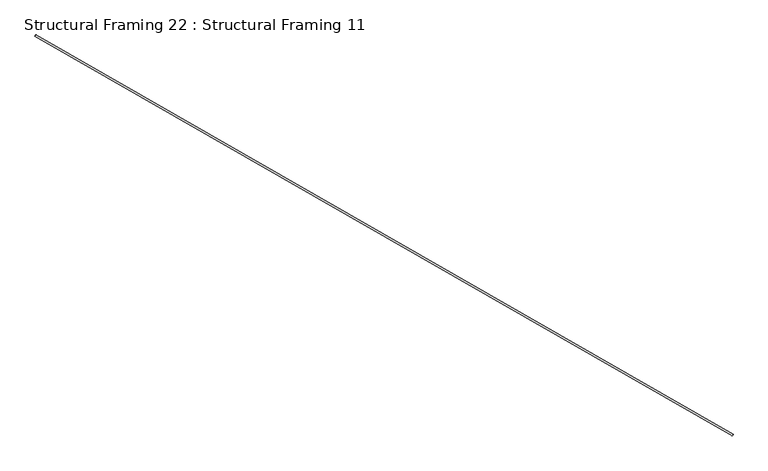
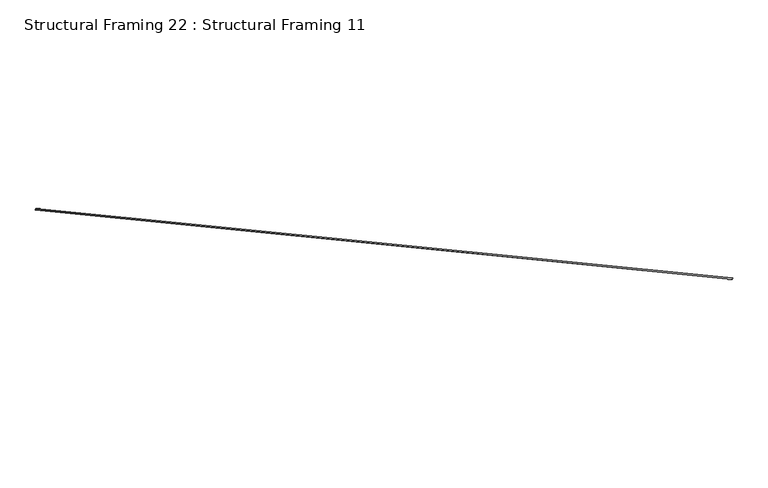
"""IFC4 building model written with IfcOpenShell, lengths in millimetres: beam geometry, Structural Framing 22 : Structural Framing 11."""

from ifc_helpers import new_model, si_unit, point, frame, origin, origin_2d, place, context, project, spatial, circle_curve, trimmed, segment, composite_curve, outline, extrude, source, transform, mapped, element, save


def structural_framing_22_structural_framing_11_913bd44a(model_context):
    return source(origin(), model_context, "Body", "SweptSolid", [
        extrude(outline(composite_curve([segment(trimmed(circle_curve(origin_2d(), 6.35), [point((0.0, -6.35))], [point((0.0, 6.35))], False, "CARTESIAN"), True, "CONTINUOUS"), segment(trimmed(circle_curve(origin_2d(), 6.35), [point((0.0, 6.35))], [point((0.0, -6.35))], False, "CARTESIAN"), True, "CONTINUOUS")], self_intersect=False)), frame((28346.1075052, 4180.6567775, 4935.1357581), z_axis=(-0.8608596592499228, 0.49364969439625245, 0.12341242359905888), x_axis=(0.0, -0.24253562503632656, 0.9701425001453335)), (0.0, 0.0, 1.0), 5892.4476777),
    ])


if __name__ == "__main__":
    model = new_model("IFC4")
    model_context = context("Model", 3, world=origin())
    ifc_project = project(units=[si_unit("LENGTHUNIT", "METRE", prefix="MILLI")], contexts=[model_context])
    site = spatial("IfcSite", under=ifc_project)
    building = spatial("IfcBuilding", under=site)
    placement = place(None, origin())
    structural_framing_22_structural_framing_11_shape = structural_framing_22_structural_framing_11_913bd44a(model_context)
    element("IfcBeam", 1, ObjectType="Structural Framing 22 : Structural Framing 11", at=placement, inside=building, context=model_context, shape_type="MappedRepresentation", body=[
        mapped(structural_framing_22_structural_framing_11_shape, transform((0.0, 0.0, 0.0), x_axis=(1.0, 0.0, 0.0), y_axis=(0.0, 1.0, 0.0), z_axis=(0.0, 0.0, 1.0))),
    ])
    save(model, "model.ifc")

# Revit data of these elements
# Type "Structural Framing 22 : Structural Framing 11"
#   Structural Material [instance default] = EXISTING LATERAL BRACING (1/4" CABLE)
# Element 1 (IfcBeam, "Structural Framing 22 : Structural Framing 11")
#   Materials on its faces: "EXISTING LATERAL BRACING (1/4\" CABLE)"
# Materials
#   "EXISTING LATERAL BRACING (1/4\" CABLE)": class "Generic", colour RGB 120 120 120, transparency 0, Cost = 0
